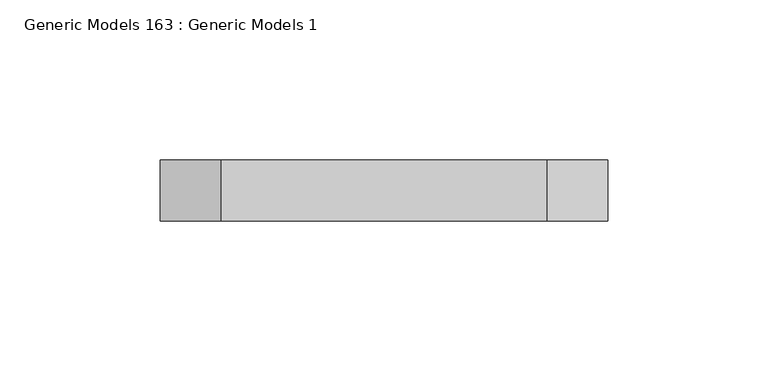
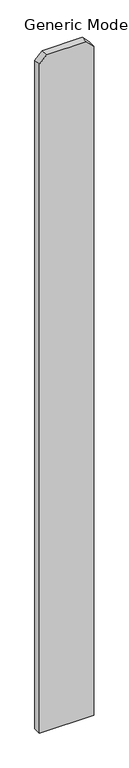
"""IFC4 building model written with IfcOpenShell, lengths in millimetres: proxy geometry, Generic Models 163 : Generic Models 1."""

from ifc_helpers import new_model, si_unit, frame, origin, place, context, project, spatial, polyline, outline, extrude, source, transform, mapped, element, save


def generic_models_163_generic_models_1_4947abff(model_context):
    return source(origin(), model_context, "Body", "SweptSolid", [
        extrude(outline(polyline([(76.2, 54837.0125), (1885.95, 54837.0125), (1905.0, 54817.9625), (1905.0, 54716.3625), (1885.95, 54697.3125), (76.2, 54697.3125), (76.2, 54837.0125)])), frame((0.0, 547.6875, 0.0), z_axis=(0.0, 1.0, 0.0), x_axis=(0.0, 0.0, 1.0)), (0.0, 0.0, 1.0), 19.05),
    ])


if __name__ == "__main__":
    model = new_model("IFC4")
    model_context = context("Model", 3, world=origin())
    ifc_project = project(units=[si_unit("LENGTHUNIT", "METRE", prefix="MILLI")], contexts=[model_context])
    site = spatial("IfcSite", under=ifc_project)
    building = spatial("IfcBuilding", under=site)
    placement = place(None, origin())
    generic_models_163_generic_models_1_shape = generic_models_163_generic_models_1_4947abff(model_context)
    element("IfcBuildingElementProxy", 1, Name="Generic Models 163 : Generic Models 1", ObjectType="Generic Models 163 : Generic Models 1", at=placement, inside=building, context=model_context, shape_type="MappedRepresentation", body=[
        mapped(generic_models_163_generic_models_1_shape, transform((0.0, 0.0, 0.0), x_axis=(1.0, 0.0, 0.0), y_axis=(0.0, 1.0, 0.0), z_axis=(0.0, 0.0, 1.0))),
    ])
    save(model, "model.ifc")

# Revit data of these elements
# Element 1 (IfcBuildingElementProxy, "Generic Models 163 : Generic Models 1")
#   Materials on its faces: "VERTICAL 1X6 CEDAR PLANKS W/ CLEAR WOOD SEALER"
# Materials
#   "VERTICAL 1X6 CEDAR PLANKS W/ CLEAR WOOD SEALER": class "Wood", colour RGB 234 198 147, transparency 0, Description = "Pinus Echinata", Cost = 0
